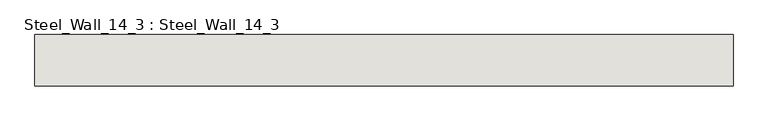
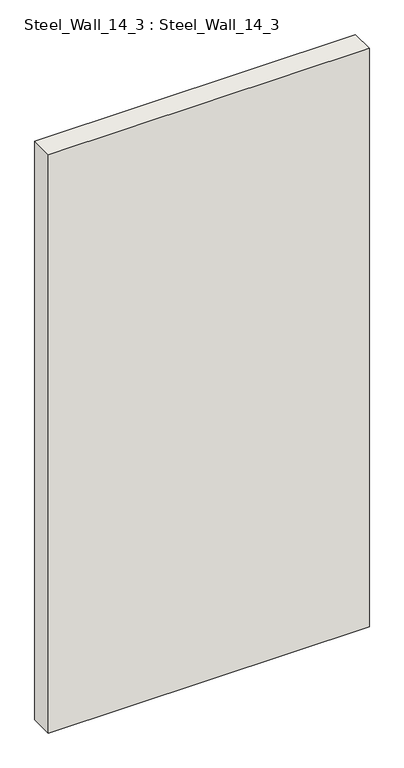
"""IFC4 building model written with IfcOpenShell, lengths in millimetres: wall geometry, Steel_Wall_14_3 : Steel_Wall_14_3."""

from ifc_helpers import new_model, si_unit, frame, origin, place, context, project, spatial, polyline, outline, extrude, source, transform, mapped, element, save


def steel_wall_14_3_steel_wall_14_3_bb8a6b82(model_context):
    return source(origin(), model_context, "Body", "SweptSolid", [
        extrude(outline(polyline([(4825.0, 395.0), (3460.0, 395.0), (3460.0, 495.0), (4825.0, 495.0), (4825.0, 395.0)])), frame((0.0, 0.0, 250.0), z_axis=(0.0, 0.0, 1.0), x_axis=(1.0, 0.0, 0.0)), (0.0, 0.0, 1.0), 2600.0),
    ])


if __name__ == "__main__":
    model = new_model("IFC4")
    model_context = context("Model", 3, world=origin())
    ifc_project = project(units=[si_unit("LENGTHUNIT", "METRE", prefix="MILLI")], contexts=[model_context])
    site = spatial("IfcSite", under=ifc_project)
    building = spatial("IfcBuilding", under=site)
    placement = place(None, origin())
    steel_wall_14_3_steel_wall_14_3_shape = steel_wall_14_3_steel_wall_14_3_bb8a6b82(model_context)
    element("IfcWall", 1, ObjectType="Steel_Wall_14_3 : Steel_Wall_14_3", at=placement, inside=building, context=model_context, shape_type="MappedRepresentation", body=[
        mapped(steel_wall_14_3_steel_wall_14_3_shape, transform((0.0, 0.0, 0.0), x_axis=(1.0, 0.0, 0.0), y_axis=(0.0, 1.0, 0.0), z_axis=(0.0, 0.0, 1.0))),
    ])
    save(model, "model.ifc")

# Revit data of these elements
# Type "Steel_Wall_14_3 : Steel_Wall_14_3"
#   NameOverride = "Steel_Wall_14_3"
# Element 1 (IfcWall, "Steel_Wall_14_3 : Steel_Wall_14_3")
#   Materials on its faces: "IfcSurfaceStyle #33"
# Materials
#   "IfcSurfaceStyle #33": class "Unassigned", colour RGB 214 214 214, transparency 0
